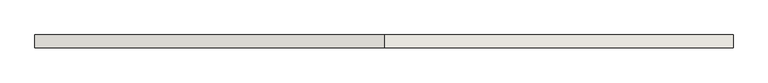
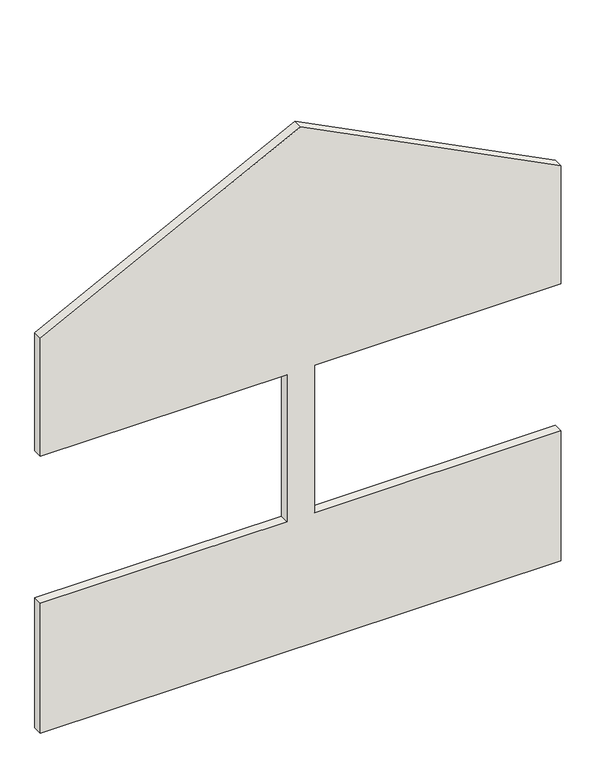
"""IFC4 building model written with IfcOpenShell, lengths in millimetres: wall geometry, 0_3d."""

from ifc_helpers import new_model, si_unit, frame, origin, place, context, project, spatial, polyline, outline, extrude, source, transform, mapped, element, save


def wall_b3749ec0(model_context):
    return source(origin(), model_context, "Body", "SweptSolid", [
        extrude(outline(polyline([(1000.0, 3800.0), (1000.0, 2000.0), (2135.0, 2000.0), (2135.0, 3800.0), (3043.5797924, 3800.0), (4011.6781465, 1900.0), (3043.5797924, 0.0), (2135.0, 0.0), (2135.0, 1800.0), (1000.0, 1800.0), (1000.0, 0.0), (0.0, 0.0), (0.0, 3800.0), (1000.0, 3800.0)])), frame((0.0, 0.0, 0.0), z_axis=(0.0, 1.0, 0.0), x_axis=(0.0, 0.0, 1.0)), (0.0, 0.0, 1.0), 70.0),
    ])


if __name__ == "__main__":
    model = new_model("IFC4")
    model_context = context("Model", 3, world=origin())
    ifc_project = project(units=[si_unit("LENGTHUNIT", "METRE", prefix="MILLI")], contexts=[model_context])
    site = spatial("IfcSite", under=ifc_project)
    building = spatial("IfcBuilding", under=site)
    placement = place(None, origin())
    wall_shape = wall_b3749ec0(model_context)
    element("IfcWall", 1, ObjectType="0_3d", at=placement, inside=building, context=model_context, shape_type="MappedRepresentation", body=[
        mapped(wall_shape, transform((0.0, 0.0, 0.0), x_axis=(1.0, 0.0, 0.0), y_axis=(0.0, 1.0, 0.0), z_axis=(0.0, 0.0, 1.0))),
    ])
    save(model, "model.ifc")

# Revit data of these elements
# Element 1 (IfcWall, "0_3d")
#   Materials on its faces: "Glass_Simple"
# Materials
#   "Glass_Simple": class "Unassigned", colour RGB 255 255 255, transparency 0.9
